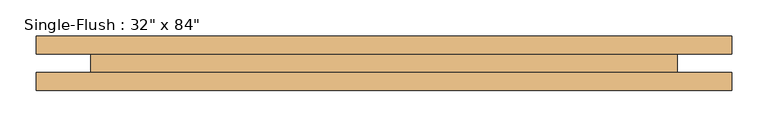
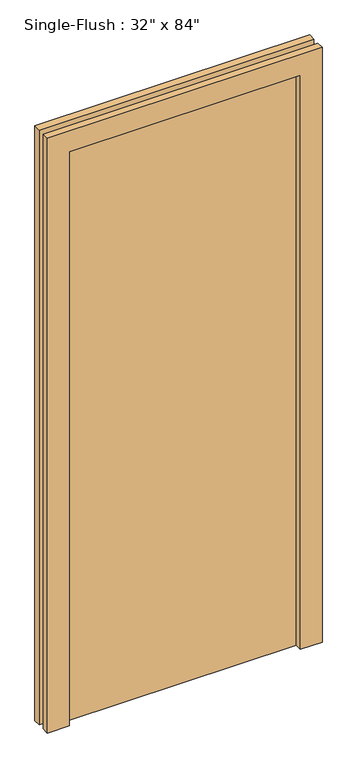
"""IFC4 building model written with IfcOpenShell, lengths in millimetres: door geometry."""

import ifcopenshell
import ifcopenshell.guid

model = None  # the IFC model being written
_history = None  # IfcOwnerHistory: only IFC2X3 demands one
_inside = {}  # id of a spatial element -> (the spatial element, [elements in it])
_under = {}  # id of a project, library or spatial element -> (it, [spatial elements below it])
_declared = {}  # id of a project -> (the project, [libraries it declares])
_typed = {}  # id of a type object -> (the type object, [elements of that type])
_made_of = {}  # id of a material, layer set ... -> (it, [elements and type objects made of it])


def new_model(schema):
    """Start an empty IFC model of exactly this schema.

    Asked for "IFC4X3", IfcOpenShell would pick the latest addendum, in which some entities
    have other attributes; the version numbers below select the first issue.
    IFC2X3 requires an IfcOwnerHistory on every rooted entity: one is made here for all.
    """
    global model, _history
    if schema == "IFC4X3":
        model = ifcopenshell.file(schema_version=(4, 3, 0, 0))
    else:
        model = ifcopenshell.file(schema=schema)
    _inside.clear()
    _under.clear()
    _declared.clear()
    _typed.clear()
    _made_of.clear()
    _history = None
    if model.schema == "IFC2X3":
        org = make("IfcOrganization", Name="unknown")
        user = make(
            "IfcPersonAndOrganization",
            ThePerson=make("IfcPerson", FamilyName="unknown"),
            TheOrganization=org,
        )
        app = make(
            "IfcApplication",
            ApplicationDeveloper=org,
            Version="unknown",
            ApplicationFullName="unknown",
            ApplicationIdentifier="unknown",
        )
        _history = make(
            "IfcOwnerHistory",
            OwningUser=user,
            OwningApplication=app,
            ChangeAction="ADDED",
            CreationDate=0,
        )
    return model


def make(cls, **values):
    """One entity of the class cls with the attributes given. An attribute that is None is left unset."""
    return model.create_entity(
        cls, **{name: value for name, value in values.items() if value is not None}
    )


def rooted(cls, **values):
    """An entity with a GlobalId (a new one), such as an element, a storey or a relation."""
    return make(cls, GlobalId=ifcopenshell.guid.new(), OwnerHistory=_history, **values)


def si_unit(unit_type, name, prefix=None):
    """IfcSIUnit, for example si_unit("LENGTHUNIT", "METRE", prefix="MILLI")."""
    return make("IfcSIUnit", UnitType=unit_type, Prefix=prefix, Name=name)


def assignment(units):
    """IfcUnitAssignment: the units of a project."""
    return None if units is None else make("IfcUnitAssignment", Units=units)


def point(xyz):
    """IfcCartesianPoint."""
    return None if xyz is None else make("IfcCartesianPoint", Coordinates=xyz)


def direction(xyz):
    """IfcDirection."""
    return None if xyz is None else make("IfcDirection", DirectionRatios=xyz)


def frame(location, z_axis=None, x_axis=None):
    """IfcAxis2Placement3D, a coordinate frame: its origin and axes. An axis left out is left unset."""
    return make(
        "IfcAxis2Placement3D",
        Location=point(location),
        Axis=direction(z_axis),
        RefDirection=direction(x_axis),
    )


def origin():
    """The frame at (0, 0, 0) with its axes left unset."""
    return frame((0.0, 0.0, 0.0))


def origin_with_axes():
    """The frame at (0, 0, 0) with the z axis (0, 0, 1) and the x axis (1, 0, 0) written out."""
    return frame((0.0, 0.0, 0.0), z_axis=(0.0, 0.0, 1.0), x_axis=(1.0, 0.0, 0.0))


def place(relative_to, where):
    """IfcLocalPlacement: puts the frame where relative to a parent placement (None: the world)."""
    return make(
        "IfcLocalPlacement", PlacementRelTo=relative_to, RelativePlacement=where
    )


def context(
    kind, dimensions, precision=None, world=None, true_north=None, identifier=None
):
    """IfcGeometricRepresentationContext, for example the 3D "Model" context."""
    return make(
        "IfcGeometricRepresentationContext",
        ContextIdentifier=identifier,
        ContextType=kind,
        CoordinateSpaceDimension=dimensions,
        Precision=precision,
        WorldCoordinateSystem=world,
        TrueNorth=true_north,
    )


def project(units=None, contexts=None):
    """IfcProject with its units and contexts."""
    return rooted(
        "IfcProject",
        Name="project",
        RepresentationContexts=contexts,
        UnitsInContext=assignment(units),
    )


def spatial(cls, under=None, at=None, **own):
    """A site, building, storey or space (cls), placed at a placement, below another one or the project."""
    s = rooted(cls, ObjectPlacement=at, **own)
    if under is not None:
        _under.setdefault(under.id(), (under, []))[1].append(s)
    return s


def polyline(points):
    """IfcPolyline through the points."""
    return make("IfcPolyline", Points=[point(p) for p in points])


def outline(outer, holes=None, kind="AREA"):
    """IfcArbitraryClosedProfileDef: a profile drawn as a closed curve; with holes, ...WithVoids."""
    if holes is None:
        return make("IfcArbitraryClosedProfileDef", ProfileType=kind, OuterCurve=outer)
    return make(
        "IfcArbitraryProfileDefWithVoids",
        ProfileType=kind,
        OuterCurve=outer,
        InnerCurves=holes,
    )


def extrude(swept, where, along, depth):
    """IfcExtrudedAreaSolid: the profile swept, set in the frame where, extruded along a direction by depth."""
    return make(
        "IfcExtrudedAreaSolid",
        SweptArea=swept,
        Position=where,
        ExtrudedDirection=direction(along),
        Depth=depth,
    )


def shape(context_of_items, identifier, shape_type, items):
    """IfcShapeRepresentation: the items that make up one representation, for example the "Body"."""
    return make(
        "IfcShapeRepresentation",
        ContextOfItems=context_of_items,
        RepresentationIdentifier=identifier,
        RepresentationType=shape_type,
        Items=items,
    )


def source(mapping_origin, context_of_items, identifier, shape_type, items):
    """IfcRepresentationMap: a shape defined once, which mapped items show again and again."""
    return make(
        "IfcRepresentationMap",
        MappingOrigin=mapping_origin,
        MappedRepresentation=shape(context_of_items, identifier, shape_type, items),
    )


def transform(
    local_origin,
    x_axis=None,
    y_axis=None,
    z_axis=None,
    scale=None,
    scale2=None,
    scale3=None,
    uniform=True,
):
    """IfcCartesianTransformationOperator3D, or its non-uniform kind. x_axis, y_axis, z_axis: its Axis1, 2, 3."""
    if uniform:
        return make(
            "IfcCartesianTransformationOperator3D",
            Axis1=direction(x_axis),
            Axis2=direction(y_axis),
            LocalOrigin=point(local_origin),
            Scale=scale,
            Axis3=direction(z_axis),
        )
    return make(
        "IfcCartesianTransformationOperator3DnonUniform",
        Axis1=direction(x_axis),
        Axis2=direction(y_axis),
        LocalOrigin=point(local_origin),
        Scale=scale,
        Axis3=direction(z_axis),
        Scale2=scale2,
        Scale3=scale3,
    )


def mapped(mapping_source, mapping_target):
    """IfcMappedItem: shows the shape of a source again, moved by a transform."""
    return make(
        "IfcMappedItem", MappingSource=mapping_source, MappingTarget=mapping_target
    )


def made_of(thing, what):
    """Note that an element or type object is made of a material, layer set ...; save() writes the relation."""
    if what is not None:
        _made_of.setdefault(what.id(), (what, []))[1].append(thing)
    return thing


def element(
    cls,
    number,
    at=None,
    inside=None,
    cuts=None,
    type_object=None,
    material=None,
    context=None,
    identifier="Body",
    shape_type=None,
    held_by="IfcProductDefinitionShape",
    body=None,
    shapes=None,
    **own,
):
    """One element of the class cls, such as IfcWall. Its Tag is "e" and its number.

    at: its placement. inside: the storey or other place that contains it. cuts: it is an
    opening in that element (IfcRelVoidsElement). A single representation is given by context,
    identifier, shape_type and body (its items); several are given by shapes. held_by: the class
    of the entity that holds the representations. save() writes the other relations.
    """
    e = rooted(cls, Tag="e%d" % number, ObjectPlacement=at, **own)
    if body is not None:
        shapes = [shape(context, identifier, shape_type, body)]
    if shapes is not None:
        e.Representation = make(held_by, Representations=shapes)
    if inside is not None:
        _inside.setdefault(inside.id(), (inside, []))[1].append(e)
    if cuts is not None:
        rooted(
            "IfcRelVoidsElement", RelatingBuildingElement=cuts, RelatedOpeningElement=e
        )
    if type_object is not None:
        _typed.setdefault(type_object.id(), (type_object, []))[1].append(e)
    return made_of(e, material)


def aggregate(whole, parts):
    """IfcRelAggregates: a whole, such as a stair, and the parts it consists of."""
    return rooted("IfcRelAggregates", RelatingObject=whole, RelatedObjects=parts)


def save(model, path):
    """Write the relations noted so far, then the file.

    IfcRelAggregates (storeys below a building ...), IfcRelContainedInSpatialStructure (elements
    in a storey), IfcRelDefinesByType, IfcRelAssociatesMaterial and IfcRelDeclares: one each for
    every whole, place, type object, material and project.
    """
    for whole, parts in _under.values():
        aggregate(whole, parts)
    for where, things in _inside.values():
        rooted(
            "IfcRelContainedInSpatialStructure",
            RelatedElements=things,
            RelatingStructure=where,
        )
    for kind, things in _typed.values():
        rooted("IfcRelDefinesByType", RelatedObjects=things, RelatingType=kind)
    for what, things in _made_of.values():
        rooted("IfcRelAssociatesMaterial", RelatedObjects=things, RelatingMaterial=what)
    for by, libraries in _declared.values():
        rooted("IfcRelDeclares", RelatingContext=by, RelatedDefinitions=libraries)
    model.write(path)


def door_5c1b3ce9(model_context):
    return source(origin(), model_context, "Body", "SweptSolid", [
        extrude(outline(polyline([(2209.8, -482.6), (0.0, -482.6), (0.0, -406.4), (2133.6, -406.4), (2133.6, 406.4), (0.0, 406.4), (0.0, 482.6), (2209.8, 482.6), (2209.8, -482.6)])), frame((0.0, -38.1, 0.0), z_axis=(0.0, 1.0, 0.0), x_axis=(0.0, 0.0, 1.0)), (0.0, 0.0, 1.0), 25.4),
        extrude(outline(polyline([(2209.8, 482.6), (2209.8, -482.6), (0.0, -482.6), (0.0, -406.4), (2133.6, -406.4), (2133.6, 406.4), (0.0, 406.4), (0.0, 482.6), (2209.8, 482.6)])), frame((0.0, 12.7, 0.0), z_axis=(0.0, 1.0, 0.0), x_axis=(0.0, 0.0, 1.0)), (0.0, 0.0, 1.0), 25.4),
        extrude(outline(polyline([(406.4, 38.1), (406.4, -12.7), (-406.4, -12.7), (-406.4, 38.1), (406.4, 38.1)])), origin_with_axes(), (0.0, 0.0, 1.0), 2133.6),
    ])


if __name__ == "__main__":
    model = new_model("IFC4")
    model_context = context("Model", 3, world=origin())
    ifc_project = project(units=[si_unit("LENGTHUNIT", "METRE", prefix="MILLI")], contexts=[model_context])
    site = spatial("IfcSite", under=ifc_project)
    building = spatial("IfcBuilding", under=site)
    placement = place(None, origin())
    door_shape = door_5c1b3ce9(model_context)
    element("IfcDoor", 1, ObjectType="Single-Flush : 32\" x 84\"", at=placement, inside=building, context=model_context, shape_type="MappedRepresentation", body=[
        mapped(door_shape, transform((0.0, 0.0, 0.0), x_axis=(1.0, 0.0, 0.0), y_axis=(0.0, 1.0, 0.0), z_axis=(0.0, 0.0, 1.0))),
    ])
    save(model, "model.ifc")

# Revit data of these elements
# Type "Single-Flush : 32\" x 84\""
#   Type Mark = "10"
#   Construction Type Id = "MDOOR"
#   Assembly Code = "C1020"
#   Analytic Construction = "Metal"
#   Thickness = 0' - 2"
#   Heat Transfer Coefficient (U) = 3.7021 W/(m²·K)
#   Height = 7' - 0"
#   Trim Projection Ext = 0' - 1"
#   Trim Projection Int = 0' - 1"
#   Trim Width = 0' - 3"
#   Width = 2' - 8"
#   Door Material = Door - Panel
#   Frame Material = Door - Frame
#   Visual Light Transmittance = 0
#   Solar Heat Gain Coefficient = 0
#   Function = (empty or 0)
#   Wall Closure = (empty or 0)
# Element 1 (IfcDoor, "Single-Flush : 32\" x 84\"")
#   Materials on its faces: "Door - Frame", "Door - Panel"
# Materials
#   "Door - Panel": class "Wood", colour RGB 210 159 95, transparency 0
#   "Door - Frame": class "Miscellaneous", colour RGB 118 70 51, transparency 0
